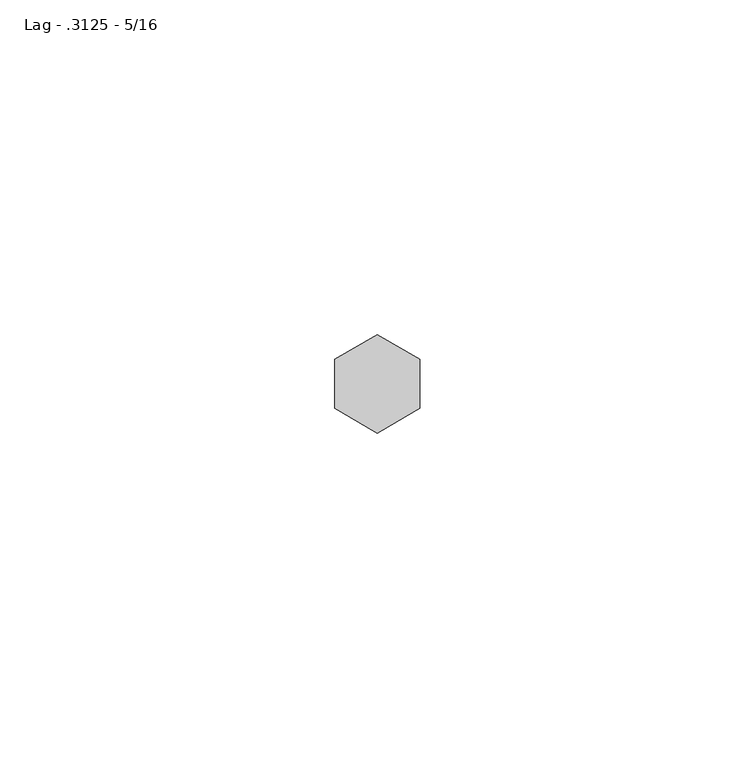
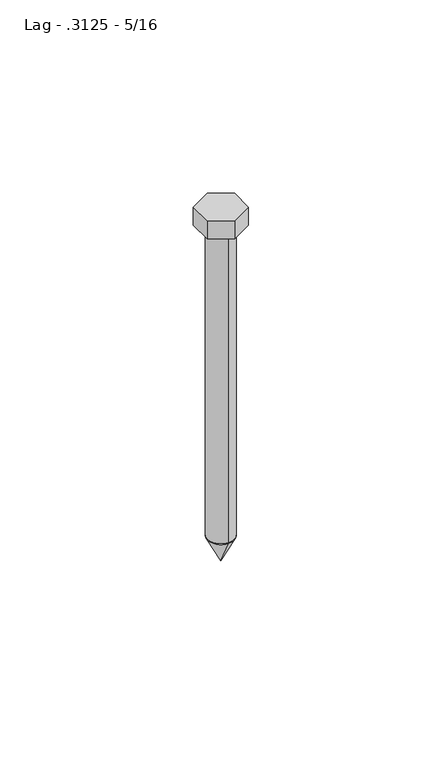
"""IFC4 building model written with IfcOpenShell, lengths in millimetres: fastener geometry, 060523 - W_P_C - Fastenings - Generic : Lag - .3125 - 5/16."""

from ifc_helpers import new_model, si_unit, point, frame, origin, origin_with_axes, origin_2d, place, context, project, spatial, polyline, circle_curve, trimmed, segment, composite_curve, outline, extrude, source, transform, mapped, element, save
from ifc_brep_helpers import plane_surface, revolved_surface, advanced_brep


def lag_3125_5_16_a232f53a(model_context):
    return source(origin(), model_context, "Body", "SolidModel", [
        advanced_brep(
        [(0.0, -4.1148, -101.6), (0.0, 4.1148, -101.6), (0.0, 0.0, -101.6), (0.0, 0.0, -109.8296)],
        [
            (0, 1, circle_curve(frame((0.0, 0.0, -101.6), z_axis=(0.0, 0.0, 1.0), x_axis=(0.0, 1.0, 0.0)), 4.1148)),
            (1, 2),
            (2, 0),
            (1, 0, circle_curve(frame((0.0, 0.0, -101.6), z_axis=(0.0, 0.0, 1.0), x_axis=(0.0, 1.0, 0.0)), 4.1148)),
            (3, 1),
            (0, 3),
        ],
        [
            plane_surface(frame((0.0, 0.0, -101.6), z_axis=(0.0, 0.0, 1.0), x_axis=(0.0, 1.0, 0.0))),
            revolved_surface(polyline([(0.0, 4.1148, -101.6), (0.0, 0.0, -109.8296)]), (0.0, 0.0, -103.0840259), (0.0, 0.0, -1.0)),
        ],
        [
            (0, [[1, 2, 3]]),
            (0, [[4, -3, -2]]),
            (1, [[5, -1, 6]]),
            (1, [[-6, -4, -5]]),
        ],
    ),
        extrude(outline(polyline([(-6.35, 3.6661742), (0.0, 7.3323484), (6.35, 3.6661742), (6.35, -3.6661742), (0.0, -7.3323484), (-6.35, -3.6661742), (-6.35, 3.6661742)])), origin_with_axes(), (0.0, 0.0, 1.0), 5.953125),
        extrude(outline(composite_curve([segment(trimmed(circle_curve(origin_2d(), 4.1148), [point((0.0, -4.1148))], [point((0.0, 4.1148))], False, "CARTESIAN"), True, "CONTINUOUS"), segment(trimmed(circle_curve(origin_2d(), 4.1148), [point((0.0, 4.1148))], [point((0.0, -4.1148))], False, "CARTESIAN"), True, "CONTINUOUS")], self_intersect=False)), frame((0.0, 0.0, -101.6), z_axis=(0.0, 0.0, 1.0), x_axis=(1.0, 0.0, 0.0)), (0.0, 0.0, 1.0), 101.6),
    ])


if __name__ == "__main__":
    model = new_model("IFC4")
    model_context = context("Model", 3, world=origin())
    ifc_project = project(units=[si_unit("LENGTHUNIT", "METRE", prefix="MILLI")], contexts=[model_context])
    site = spatial("IfcSite", under=ifc_project)
    building = spatial("IfcBuilding", under=site)
    placement = place(None, origin())
    lag_3125_5_16_shape = lag_3125_5_16_a232f53a(model_context)
    element("IfcFastener", 1, ObjectType="060523 - W_P_C - Fastenings - Generic : Lag - .3125 - 5/16", at=placement, inside=building, context=model_context, shape_type="MappedRepresentation", body=[
        mapped(lag_3125_5_16_shape, transform((0.0, 0.0, 0.0), x_axis=(1.0, 0.0, 0.0), y_axis=(0.0, 1.0, 0.0), z_axis=(0.0, 0.0, 1.0))),
    ])
    save(model, "model.ifc")

# Revit data of these elements
# Type "060523 - W_P_C - Fastenings - Generic : Lag - .3125 - 5/16"
#   Washer_Thickness = 0' - 0 5/64"
#   Washer Radius = 0' - 0.39638"
#   Washer Offset - Head = 0' - 0"
#   Washer Offset = 0' - 0"
#   Thickness_of_Substrate [instance default] = 0' - 1"
#   Side = 0' - 0 37/128"
#   Radius = 0' - 0.162"
#   Length [instance default] = 0' - 4"
#   Head Size = 0' - 0 1/2"
#   Head Radius = 0' - 0 1/4"
#   Head Height = 0' - 0 15/64"
#   Double Diameter = 0' - 0.648"
#   Diameter = 0' - 0.324"
#   Default Elevation = 4' - 0"
#   Washer_Nut_Visibility = no
#   Washer_Head_Visibility = no
#   Round_Head_Visibility = no
#   Point Visibility = yes
#   Nut_Visibility = no
#   Hex_Head_Visiblilty = yes
#   Washer Material = none
#   Bolt Material (Size) = AT SILL - FASTENER AT 24" O.C.
# Element 1 (IfcFastener, "060523 - W_P_C - Fastenings - Generic : Lag - .3125 - 5/16")
#   Materials on its faces: "AT SILL - FASTENER AT 24\" O.C."
# Materials
#   "AT SILL - FASTENER AT 24\" O.C.": class "Generic", colour RGB 120 120 120, transparency 0, Cost = 0
